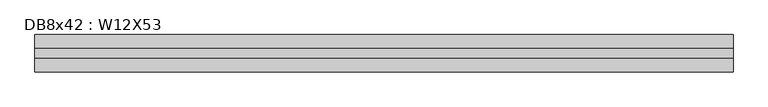
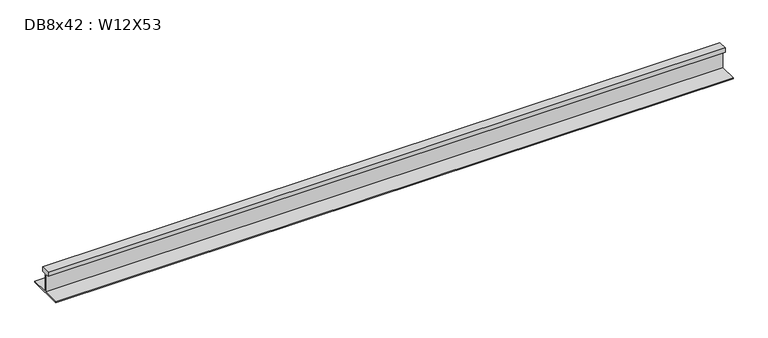
"""IFC4 building model written with IfcOpenShell, lengths in millimetres: beam geometry, DB8x42 : W12X53."""

from ifc_helpers import new_model, si_unit, frame, origin, place, context, project, spatial, polyline, outline, extrude, source, transform, mapped, element, save


def db8x42_w12x53_04ca51d8(model_context):
    return source(origin(), model_context, "Body", "SweptSolid", [
        extrude(outline(polyline([(38.1, 144.3355), (38.1, 106.2355), (4.7625, 106.2355), (4.7625, -49.53), (152.4, -49.53), (152.4, -59.182), (-152.4, -59.182), (-152.4, -49.53), (-4.7625, -49.53), (-4.7625, 106.2355), (-38.1, 106.2355), (-38.1, 144.3355), (38.1, 144.3355)])), frame((-2844.8, 0.0, 0.0), z_axis=(1.0, 0.0, 0.0), x_axis=(0.0, 1.0, 0.0)), (0.0, 0.0, 1.0), 5676.8999994),
    ])


if __name__ == "__main__":
    model = new_model("IFC4")
    model_context = context("Model", 3, world=origin())
    ifc_project = project(units=[si_unit("LENGTHUNIT", "METRE", prefix="MILLI")], contexts=[model_context])
    site = spatial("IfcSite", under=ifc_project)
    building = spatial("IfcBuilding", under=site)
    placement = place(None, origin())
    db8x42_w12x53_shape = db8x42_w12x53_04ca51d8(model_context)
    element("IfcBeam", 1, ObjectType="DB8x42 : W12X53", at=placement, inside=building, context=model_context, shape_type="MappedRepresentation", body=[
        mapped(db8x42_w12x53_shape, transform((0.0, 0.0, 0.0), x_axis=(1.0, 0.0, 0.0), y_axis=(0.0, 1.0, 0.0), z_axis=(0.0, 0.0, 1.0))),
    ])
    save(model, "model.ifc")

# Revit data of these elements
# Type "DB8x42 : W12X53"
#   Assembly Code = "B10"
#   W = 53
#   Length [instance default] = 5' - 0"
#   bf = 0' - 10"
#   d = 1' - 0.1"
#   k = 0' - 1 3/8"
#   k2 = 0' - 0.8"
#   tf = 0' - 0.575"
#   tw = 0' - 0.345"
#   A = 0.108333 SF
#   Structural Material [instance default] = Steel ASTM A992
# Element 1 (IfcBeam, "DB8x42 : W12X53")
#   Materials on its faces: "Steel ASTM A992"
# Materials
#   "Steel ASTM A992": class "Metal", colour RGB 199 199 199, transparency 0, Description = "Structural steel 50ksi", Cost = 0
